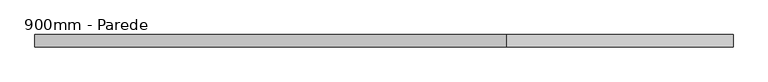
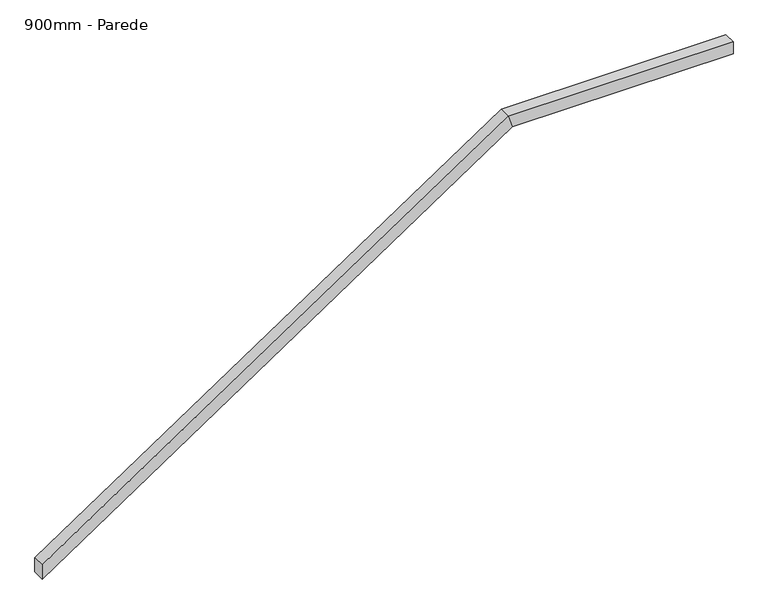
"""IFC4 building model written with IfcOpenShell, lengths in millimetres: railing geometry, 900mm - Parede."""

from ifc_helpers import new_model, si_unit, origin, place, context, project, spatial, faceted_brep, source, transform, mapped, element, save


def railing_900mm_parede_024ee174(model_context):
    return source(origin(), model_context, "Body", "Brep", [
        faceted_brep([(-1668.4017601, 707.3270982, 1480.0), (-1668.4017601, 707.3270982, 1419.9074787), (-1668.4017601, 657.3270982, 1419.9074787), (-1668.4017601, 657.3270982, 1480.0), (221.5982399, 707.3270982, 2740.0), (236.7370218, 707.3270982, 2690.0), (236.7370218, 657.3270982, 2690.0), (221.5982399, 657.3270982, 2740.0), (1131.5982399, 707.3270982, 2740.0), (1131.5982399, 657.3270982, 2740.0), (1131.5982399, 657.3270982, 2690.0), (1131.5982399, 707.3270982, 2690.0)], [[[0, 1, 2, 3]], [[1, 0, 4, 5]], [[2, 1, 5, 6]], [[3, 2, 6, 7]], [[0, 3, 7, 4]], [[8, 9, 10, 11]], [[5, 4, 8, 11]], [[6, 5, 11, 10]], [[7, 6, 10, 9]], [[4, 7, 9, 8]]]),
    ])


if __name__ == "__main__":
    model = new_model("IFC4")
    model_context = context("Model", 3, world=origin())
    ifc_project = project(units=[si_unit("LENGTHUNIT", "METRE", prefix="MILLI")], contexts=[model_context])
    site = spatial("IfcSite", under=ifc_project)
    building = spatial("IfcBuilding", under=site)
    placement = place(None, origin())
    railing_900mm_parede_shape = railing_900mm_parede_024ee174(model_context)
    element("IfcRailing", 1, ObjectType="900mm - Parede", at=placement, inside=building, context=model_context, shape_type="MappedRepresentation", body=[
        mapped(railing_900mm_parede_shape, transform((0.0, 0.0, 0.0), x_axis=(1.0, 0.0, 0.0), y_axis=(0.0, 1.0, 0.0), z_axis=(0.0, 0.0, 1.0))),
    ])
    save(model, "model.ifc")

# Revit data of these elements
# Element 1 (IfcRailing, "900mm - Parede")
#   Materials on its faces: ".MADEIRAMENTO"
# Materials
#   ".MADEIRAMENTO": class ".CC_MADEIRAS", colour RGB 212 179 113, transparency 0, Cost = 0
